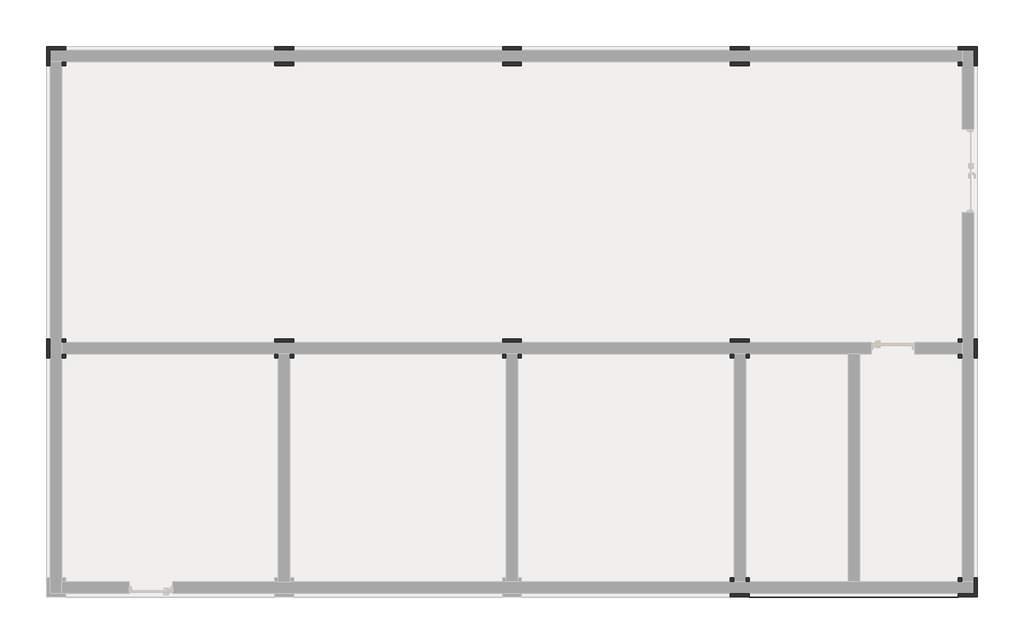
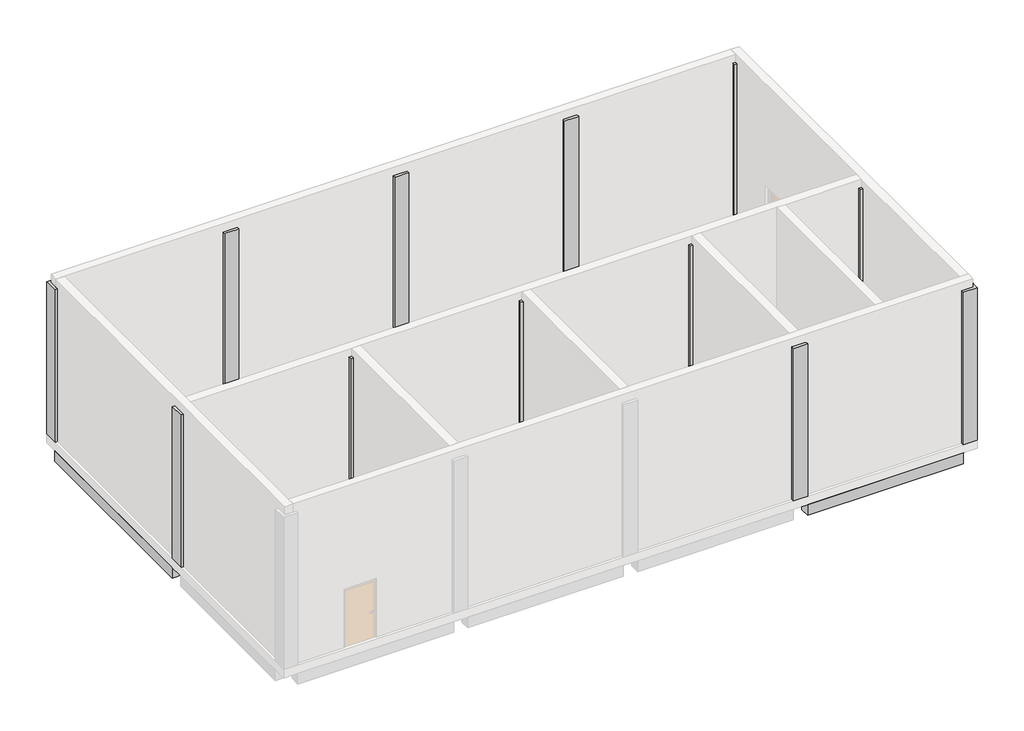
# One storey, part 2 of 2: 12 columns, 8 beams.
"""IFC4 building model written with IfcOpenShell, lengths in millimetres."""

import ifcopenshell
import ifcopenshell.guid

model = None  # the IFC model being written
_history = None  # IfcOwnerHistory: only IFC2X3 demands one
_inside = {}  # id of a spatial element -> (the spatial element, [elements in it])
_under = {}  # id of a project, library or spatial element -> (it, [spatial elements below it])
_declared = {}  # id of a project -> (the project, [libraries it declares])
_typed = {}  # id of a type object -> (the type object, [elements of that type])
_made_of = {}  # id of a material, layer set ... -> (it, [elements and type objects made of it])


def new_model(schema):
    """Start an empty IFC model of exactly this schema.

    Asked for "IFC4X3", IfcOpenShell would pick the latest addendum, in which some entities
    have other attributes; the version numbers below select the first issue.
    IFC2X3 requires an IfcOwnerHistory on every rooted entity: one is made here for all.
    """
    global model, _history
    if schema == "IFC4X3":
        model = ifcopenshell.file(schema_version=(4, 3, 0, 0))
    else:
        model = ifcopenshell.file(schema=schema)
    _inside.clear()
    _under.clear()
    _declared.clear()
    _typed.clear()
    _made_of.clear()
    _history = None
    if model.schema == "IFC2X3":
        org = make("IfcOrganization", Name="unknown")
        user = make(
            "IfcPersonAndOrganization",
            ThePerson=make("IfcPerson", FamilyName="unknown"),
            TheOrganization=org,
        )
        app = make(
            "IfcApplication",
            ApplicationDeveloper=org,
            Version="unknown",
            ApplicationFullName="unknown",
            ApplicationIdentifier="unknown",
        )
        _history = make(
            "IfcOwnerHistory",
            OwningUser=user,
            OwningApplication=app,
            ChangeAction="ADDED",
            CreationDate=0,
        )
    return model


def make(cls, **values):
    """One entity of the class cls with the attributes given. An attribute that is None is left unset."""
    return model.create_entity(
        cls, **{name: value for name, value in values.items() if value is not None}
    )


def rooted(cls, **values):
    """An entity with a GlobalId (a new one), such as an element, a storey or a relation."""
    return make(cls, GlobalId=ifcopenshell.guid.new(), OwnerHistory=_history, **values)


def si_unit(unit_type, name, prefix=None):
    """IfcSIUnit, for example si_unit("LENGTHUNIT", "METRE", prefix="MILLI")."""
    return make("IfcSIUnit", UnitType=unit_type, Prefix=prefix, Name=name)


def assignment(units):
    """IfcUnitAssignment: the units of a project."""
    return None if units is None else make("IfcUnitAssignment", Units=units)


def point(xyz):
    """IfcCartesianPoint."""
    return None if xyz is None else make("IfcCartesianPoint", Coordinates=xyz)


def direction(xyz):
    """IfcDirection."""
    return None if xyz is None else make("IfcDirection", DirectionRatios=xyz)


def frame(location, z_axis=None, x_axis=None):
    """IfcAxis2Placement3D, a coordinate frame: its origin and axes. An axis left out is left unset."""
    return make(
        "IfcAxis2Placement3D",
        Location=point(location),
        Axis=direction(z_axis),
        RefDirection=direction(x_axis),
    )


def origin():
    """The frame at (0, 0, 0) with its axes left unset."""
    return frame((0.0, 0.0, 0.0))


def place(relative_to, where):
    """IfcLocalPlacement: puts the frame where relative to a parent placement (None: the world)."""
    return make(
        "IfcLocalPlacement", PlacementRelTo=relative_to, RelativePlacement=where
    )


def context(
    kind, dimensions, precision=None, world=None, true_north=None, identifier=None
):
    """IfcGeometricRepresentationContext, for example the 3D "Model" context."""
    return make(
        "IfcGeometricRepresentationContext",
        ContextIdentifier=identifier,
        ContextType=kind,
        CoordinateSpaceDimension=dimensions,
        Precision=precision,
        WorldCoordinateSystem=world,
        TrueNorth=true_north,
    )


def project(units=None, contexts=None):
    """IfcProject with its units and contexts."""
    return rooted(
        "IfcProject",
        Name="project",
        RepresentationContexts=contexts,
        UnitsInContext=assignment(units),
    )


def spatial(cls, under=None, at=None, **own):
    """A site, building, storey or space (cls), placed at a placement, below another one or the project."""
    s = rooted(cls, ObjectPlacement=at, **own)
    if under is not None:
        _under.setdefault(under.id(), (under, []))[1].append(s)
    return s


def polyline(points):
    """IfcPolyline through the points."""
    return make("IfcPolyline", Points=[point(p) for p in points])


def outline(outer, holes=None, kind="AREA"):
    """IfcArbitraryClosedProfileDef: a profile drawn as a closed curve; with holes, ...WithVoids."""
    if holes is None:
        return make("IfcArbitraryClosedProfileDef", ProfileType=kind, OuterCurve=outer)
    return make(
        "IfcArbitraryProfileDefWithVoids",
        ProfileType=kind,
        OuterCurve=outer,
        InnerCurves=holes,
    )


def extrude(swept, where, along, depth):
    """IfcExtrudedAreaSolid: the profile swept, set in the frame where, extruded along a direction by depth."""
    return make(
        "IfcExtrudedAreaSolid",
        SweptArea=swept,
        Position=where,
        ExtrudedDirection=direction(along),
        Depth=depth,
    )


def faces_of(points, faces, orient=None, outer=None):
    """IfcFace entities. A face is a list of loops; a loop is a list of indices into points, from 0.

    orient and outer hold one flag for each loop. By default every Orientation is true, the
    first loop of a face is its IfcFaceOuterBound and the others are IfcFaceBound.
    """
    made = []
    for i, loops in enumerate(faces):
        bounds = []
        for j, loop in enumerate(loops):
            is_outer = j == 0 if outer is None else outer[i][j]
            bounds.append(
                make(
                    "IfcFaceOuterBound" if is_outer else "IfcFaceBound",
                    Bound=make("IfcPolyLoop", Polygon=[points[k] for k in loop]),
                    Orientation=True if orient is None else orient[i][j],
                )
            )
        made.append(make("IfcFace", Bounds=bounds))
    return made


def faceted_brep(points, faces, orient=None, outer=None, voids=None):
    """IfcFacetedBrep: a solid bounded by flat faces; with voids (closed shells), ...WithVoids."""
    shared = [point(p) for p in points]
    hull = make("IfcClosedShell", CfsFaces=faces_of(shared, faces, orient, outer))
    if voids is None:
        return make("IfcFacetedBrep", Outer=hull)
    return make(
        "IfcFacetedBrepWithVoids",
        Outer=hull,
        Voids=[
            make(cls, CfsFaces=faces_of(shared, fs, o, b)) for cls, fs, o, b in voids
        ],
    )


def shape(context_of_items, identifier, shape_type, items):
    """IfcShapeRepresentation: the items that make up one representation, for example the "Body"."""
    return make(
        "IfcShapeRepresentation",
        ContextOfItems=context_of_items,
        RepresentationIdentifier=identifier,
        RepresentationType=shape_type,
        Items=items,
    )


def made_of(thing, what):
    """Note that an element or type object is made of a material, layer set ...; save() writes the relation."""
    if what is not None:
        _made_of.setdefault(what.id(), (what, []))[1].append(thing)
    return thing


def element(
    cls,
    number,
    at=None,
    inside=None,
    cuts=None,
    type_object=None,
    material=None,
    context=None,
    identifier="Body",
    shape_type=None,
    held_by="IfcProductDefinitionShape",
    body=None,
    shapes=None,
    **own,
):
    """One element of the class cls, such as IfcWall. Its Tag is "e" and its number.

    at: its placement. inside: the storey or other place that contains it. cuts: it is an
    opening in that element (IfcRelVoidsElement). A single representation is given by context,
    identifier, shape_type and body (its items); several are given by shapes. held_by: the class
    of the entity that holds the representations. save() writes the other relations.
    """
    e = rooted(cls, Tag="e%d" % number, ObjectPlacement=at, **own)
    if body is not None:
        shapes = [shape(context, identifier, shape_type, body)]
    if shapes is not None:
        e.Representation = make(held_by, Representations=shapes)
    if inside is not None:
        _inside.setdefault(inside.id(), (inside, []))[1].append(e)
    if cuts is not None:
        rooted(
            "IfcRelVoidsElement", RelatingBuildingElement=cuts, RelatedOpeningElement=e
        )
    if type_object is not None:
        _typed.setdefault(type_object.id(), (type_object, []))[1].append(e)
    return made_of(e, material)


def aggregate(whole, parts):
    """IfcRelAggregates: a whole, such as a stair, and the parts it consists of."""
    return rooted("IfcRelAggregates", RelatingObject=whole, RelatedObjects=parts)


def save(model, path):
    """Write the relations noted so far, then the file.

    IfcRelAggregates (storeys below a building ...), IfcRelContainedInSpatialStructure (elements
    in a storey), IfcRelDefinesByType, IfcRelAssociatesMaterial and IfcRelDeclares: one each for
    every whole, place, type object, material and project.
    """
    for whole, parts in _under.values():
        aggregate(whole, parts)
    for where, things in _inside.values():
        rooted(
            "IfcRelContainedInSpatialStructure",
            RelatedElements=things,
            RelatingStructure=where,
        )
    for kind, things in _typed.values():
        rooted("IfcRelDefinesByType", RelatedObjects=things, RelatingType=kind)
    for what, things in _made_of.values():
        rooted("IfcRelAssociatesMaterial", RelatedObjects=things, RelatingMaterial=what)
    for by, libraries in _declared.values():
        rooted("IfcRelDeclares", RelatingContext=by, RelatedDefinitions=libraries)
    model.write(path)


model = new_model("IFC4")

# Units and contexts
model_context = context("Model", 3, world=origin())
ifc_project = project(units=[si_unit("LENGTHUNIT", "METRE", prefix="MILLI")], contexts=[model_context])

# Site, building, storey
site = spatial("IfcSite", under=ifc_project)
building = spatial("IfcBuilding", under=site)
storey = spatial("IfcBuildingStorey", under=building, Name="1st FL GL+200", Elevation=0.0)

# Beams
placement = place(None, origin())
element("IfcBeam", 1, ObjectType="RC Beam_Rectangular : 350 x 700mm", at=placement, inside=storey, context=model_context, shape_type="SweptSolid", body=[
    extrude(outline(polyline([(5204.2726763, 1485.9763125), (5554.2726763, 1485.9763125), (5554.2726763, -4314.0236875), (5204.2726763, -4314.0236875), (5204.2726763, 1485.9763125)])), frame((0.0, 0.0, -700.0), z_axis=(0.0, 0.0, 1.0), x_axis=(1.0, 0.0, 0.0)), (0.0, 0.0, 1.0), 400.0),
])
element("IfcBeam", 2, ObjectType="RC Beam_Rectangular : 350 x 700mm", at=placement, inside=storey, context=model_context, shape_type="SweptSolid", body=[
    extrude(outline(polyline([(5554.2726763, 1998.6763125), (5204.2726763, 1998.6763125), (5204.2726763, 9185.9763125), (5554.2726763, 9185.9763125), (5554.2726763, 1998.6763125)])), frame((0.0, 0.0, -700.0), z_axis=(0.0, 0.0, 1.0), x_axis=(1.0, 0.0, 0.0)), (0.0, 0.0, 1.0), 400.0),
])
element("IfcBeam", 3, ObjectType="RC Beam_Rectangular : 350 x 700mm", at=placement, inside=storey, context=model_context, shape_type="SweptSolid", body=[
    extrude(outline(polyline([(-18595.7273237, 1998.6763125), (-18945.7273237, 1998.6763125), (-18945.7273237, 9185.9763125), (-18595.7273237, 9185.9763125), (-18595.7273237, 1998.6763125)])), frame((0.0, 0.0, -700.0), z_axis=(0.0, 0.0, 1.0), x_axis=(1.0, 0.0, 0.0)), (0.0, 0.0, 1.0), 400.0),
])
element("IfcBeam", 4, ObjectType="RC Beam_Rectangular : 350 x 700mm", at=placement, inside=storey, context=model_context, shape_type="SweptSolid", body=[
    extrude(outline(polyline([(-12945.7273237, 9685.9763125), (-12945.7273237, 9335.9763125), (-18445.7273237, 9335.9763125), (-18445.7273237, 9685.9763125), (-12945.7273237, 9685.9763125)])), frame((0.0, 0.0, -700.0), z_axis=(0.0, 0.0, 1.0), x_axis=(1.0, 0.0, 0.0)), (0.0, 0.0, 1.0), 400.0),
])
element("IfcBeam", 5, ObjectType="RC Beam_Rectangular : 350 x 700mm", at=placement, inside=storey, context=model_context, shape_type="SweptSolid", body=[
    extrude(outline(polyline([(-12433.0273237, 9335.9763125), (-12433.0273237, 9685.9763125), (-6945.7273237, 9685.9763125), (-6945.7273237, 9335.9763125), (-12433.0273237, 9335.9763125)])), frame((0.0, 0.0, -700.0), z_axis=(0.0, 0.0, 1.0), x_axis=(1.0, 0.0, 0.0)), (0.0, 0.0, 1.0), 400.0),
])
element("IfcBeam", 6, ObjectType="RC Beam_Rectangular : 350 x 700mm", at=placement, inside=storey, context=model_context, shape_type="SweptSolid", body=[
    extrude(outline(polyline([(-6433.0273237, 9335.9763125), (-6433.0273237, 9685.9763125), (-945.7273237, 9685.9763125), (-945.7273237, 9335.9763125), (-6433.0273237, 9335.9763125)])), frame((0.0, 0.0, -700.0), z_axis=(0.0, 0.0, 1.0), x_axis=(1.0, 0.0, 0.0)), (0.0, 0.0, 1.0), 400.0),
])
element("IfcBeam", 7, ObjectType="RC Beam_Rectangular : 350 x 700mm", at=placement, inside=storey, context=model_context, shape_type="SweptSolid", body=[
    extrude(outline(polyline([(-433.0273237, 9335.9763125), (-433.0273237, 9685.9763125), (5054.2726763, 9685.9763125), (5054.2726763, 9335.9763125), (-433.0273237, 9335.9763125)])), frame((0.0, 0.0, -700.0), z_axis=(0.0, 0.0, 1.0), x_axis=(1.0, 0.0, 0.0)), (0.0, 0.0, 1.0), 400.0),
])
element("IfcBeam", 8, ObjectType="RC Beam_Rectangular : 350 x 700mm", at=placement, inside=storey, context=model_context, shape_type="SweptSolid", body=[
    extrude(outline(polyline([(5054.2726763, -4464.0236875), (5054.2726763, -4814.0236875), (-445.7273237, -4814.0236875), (-445.7273237, -4464.0236875), (5054.2726763, -4464.0236875)])), frame((0.0, 0.0, -700.0), z_axis=(0.0, 0.0, 1.0), x_axis=(1.0, 0.0, 0.0)), (0.0, 0.0, 1.0), 400.0),
])

# Columns
element("IfcColumn", 9, ObjectType="RC_Column_Rectangular : 500 x 500mm", at=placement, inside=storey, context=model_context, shape_type="Brep", body=[
    faceted_brep([(-18945.7273237, 9185.9763125, 0.0), (-18945.7273237, 9685.9763125, 0.0), (-18445.7273237, 9685.9763125, 0.0), (-18445.7273237, 9585.9763125, 0.0), (-18845.7273237, 9585.9763125, 0.0), (-18845.7273237, 9285.9763125, 0.0), (-18845.7273237, 9185.9763125, 0.0), (-18945.7273237, 9685.9763125, 5700.0), (-18445.7273237, 9685.9763125, 5700.0), (-18445.7273237, 9685.9763125, 5300.0), (-18945.7273237, 9185.9763125, 5300.0), (-18945.7273237, 9185.9763125, 5700.0), (-18845.7273237, 9185.9763125, 5300.0), (-18845.7273237, 9185.9763125, 5700.0), (-18445.7273237, 9585.9763125, 5700.0), (-18445.7273237, 9585.9763125, 5300.0), (-18845.7273237, 9585.9763125, 5700.0)], [[[0, 1, 2, 3, 4, 5, 6]], [[2, 1, 7, 8, 9]], [[1, 0, 10, 11, 7]], [[11, 10, 0, 6, 12, 13]], [[2, 9, 8, 14, 15, 3]], [[16, 4, 3, 15, 14]], [[4, 16, 13, 12, 6, 5]], [[8, 7, 11, 13, 16, 14]]]),
    faceted_brep([(-18445.7273237, 9185.9763125, 5700.0), (-18445.7273237, 9285.9763125, 5700.0), (-18545.7273237, 9285.9763125, 5700.0), (-18545.7273237, 9185.9763125, 5700.0), (-18445.7273237, 9285.9763125, 0.0), (-18545.7273237, 9285.9763125, 0.0), (-18445.7273237, 9185.9763125, 0.0), (-18545.7273237, 9185.9763125, 0.0)], [[[0, 1, 2, 3]], [[1, 4, 5, 2]], [[0, 6, 4, 1]], [[5, 7, 3, 2]], [[4, 6, 7, 5]], [[6, 0, 3, 7]]]),
])
element("IfcColumn", 10, ObjectType="RC_Column_Rectangular : 500 x 500mm", at=placement, inside=storey, context=model_context, shape_type="Brep", body=[
    faceted_brep([(-18945.7273237, 1485.9763125, 0.0), (-18945.7273237, 1985.9763125, 0.0), (-18845.7273237, 1985.9763125, 0.0), (-18845.7273237, 1485.9763125, 0.0), (-18945.7273237, 1485.9763125, 5300.0), (-18945.7273237, 1485.9763125, 5700.0), (-18945.7273237, 1985.9763125, 5700.0), (-18945.7273237, 1985.9763125, 5300.0), (-18845.7273237, 1485.9763125, 5300.0), (-18845.7273237, 1485.9763125, 5700.0), (-18845.7273237, 1985.9763125, 5300.0), (-18845.7273237, 1985.9763125, 5700.0)], [[[0, 1, 2, 3]], [[1, 0, 4, 5, 6, 7]], [[5, 4, 0, 3, 8, 9]], [[3, 2, 10, 11, 9, 8]], [[1, 7, 6, 11, 10, 2]], [[6, 5, 9, 11]]]),
    faceted_brep([(-18445.7273237, 1985.9763125, 5700.0), (-18445.7273237, 1985.9763125, 0.0), (-18545.7273237, 1985.9763125, 0.0), (-18545.7273237, 1985.9763125, 5700.0), (-18445.7273237, 1910.9763125, 5700.0), (-18445.7273237, 1885.9763125, 5700.0), (-18445.7273237, 1885.9763125, 5300.0), (-18445.7273237, 1885.9763125, 0.0), (-18545.7273237, 1885.9763125, 0.0), (-18545.7273237, 1885.9763125, 5700.0)], [[[0, 1, 2, 3]], [[1, 0, 4, 5, 6, 7]], [[2, 1, 7, 8]], [[7, 6, 5, 9, 8]], [[0, 3, 9, 5, 4]], [[3, 2, 8, 9]]]),
    faceted_brep([(-18545.7273237, 1485.9763125, 5700.0), (-18445.7273237, 1485.9763125, 5700.0), (-18445.7273237, 1560.9763125, 5700.0), (-18445.7273237, 1585.9763125, 5700.0), (-18545.7273237, 1585.9763125, 5700.0), (-18545.7273237, 1485.9763125, 0.0), (-18545.7273237, 1585.9763125, 0.0), (-18445.7273237, 1485.9763125, 0.0), (-18445.7273237, 1585.9763125, 5300.0), (-18445.7273237, 1585.9763125, 0.0)], [[[0, 1, 2, 3, 4]], [[5, 0, 4, 6]], [[7, 1, 0, 5]], [[3, 8, 9, 6, 4]], [[1, 7, 9, 8, 3, 2]], [[7, 5, 6, 9]]]),
])
element("IfcColumn", 11, ObjectType="RC_Column_Rectangular : 500 x 500mm", at=placement, inside=storey, context=model_context, shape_type="Brep", body=[
    faceted_brep([(-12945.7273237, 9685.9763125, 0.0), (-12445.7273237, 9685.9763125, 0.0), (-12445.7273237, 9585.9763125, 0.0), (-12945.7273237, 9585.9763125, 0.0), (-12945.7273237, 9685.9763125, 5300.0), (-12945.7273237, 9685.9763125, 5700.0), (-12445.7273237, 9685.9763125, 5700.0), (-12945.7273237, 9585.9763125, 5300.0), (-12945.7273237, 9585.9763125, 5700.0), (-12445.7273237, 9585.9763125, 5700.0)], [[[0, 1, 2, 3]], [[1, 0, 4, 5, 6]], [[5, 4, 0, 3, 7, 8]], [[1, 6, 9, 2]], [[3, 2, 9, 8, 7]], [[6, 5, 8, 9]]]),
    faceted_brep([(-12945.7273237, 9185.9763125, 0.0), (-12445.7273237, 9185.9763125, 0.0), (-12445.7273237, 9185.9763125, 5700.0), (-12520.7273237, 9185.9763125, 5700.0), (-12870.7273237, 9185.9763125, 5700.0), (-12945.7273237, 9185.9763125, 5700.0), (-12445.7273237, 9285.9763125, 5700.0), (-12945.7273237, 9285.9763125, 5700.0), (-12445.7273237, 9285.9763125, 0.0), (-12945.7273237, 9285.9763125, 0.0)], [[[0, 1, 2, 3, 4, 5]], [[5, 4, 3, 2, 6, 7]], [[8, 9, 7, 6]], [[1, 0, 9, 8]], [[0, 5, 7, 9]], [[2, 1, 8, 6]]]),
])
element("IfcColumn", 12, ObjectType="RC_Column_Rectangular : 500 x 500mm", at=placement, inside=storey, context=model_context, shape_type="Brep", body=[
    faceted_brep([(-12945.7273237, 1985.9763125, 0.0), (-12445.7273237, 1985.9763125, 0.0), (-12445.7273237, 1885.9763125, 0.0), (-12945.7273237, 1885.9763125, 0.0), (-12945.7273237, 1985.9763125, 5700.0), (-12870.7273237, 1985.9763125, 5700.0), (-12520.7273237, 1985.9763125, 5700.0), (-12445.7273237, 1985.9763125, 5700.0), (-12945.7273237, 1885.9763125, 5300.0), (-12945.7273237, 1885.9763125, 5700.0), (-12945.7273237, 1910.9763125, 5700.0), (-12445.7273237, 1910.9763125, 5700.0), (-12445.7273237, 1885.9763125, 5700.0), (-12445.7273237, 1885.9763125, 5300.0)], [[[0, 1, 2, 3]], [[1, 0, 4, 5, 6, 7]], [[4, 0, 3, 8, 9, 10]], [[1, 7, 11, 12, 13, 2]], [[3, 2, 13, 12, 9, 8]], [[7, 6, 5, 4, 10, 9, 12, 11]]]),
    faceted_brep([(-12945.7273237, 1485.9763125, 5700.0), (-12945.7273237, 1485.9763125, 0.0), (-12845.7273237, 1485.9763125, 0.0), (-12845.7273237, 1485.9763125, 5300.0), (-12845.7273237, 1485.9763125, 5700.0), (-12870.7273237, 1485.9763125, 5700.0), (-12945.7273237, 1585.9763125, 0.0), (-12945.7273237, 1585.9763125, 5300.0), (-12945.7273237, 1585.9763125, 5700.0), (-12845.7273237, 1585.9763125, 5700.0), (-12845.7273237, 1585.9763125, 0.0), (-12945.7273237, 1560.9763125, 5700.0)], [[[0, 1, 2, 3, 4, 5]], [[6, 7, 8, 9, 10]], [[1, 6, 10, 2]], [[1, 0, 11, 8, 7, 6]], [[4, 3, 2, 10, 9]], [[8, 11, 0, 5, 4, 9]]]),
    faceted_brep([(-12445.7273237, 1485.9763125, 5700.0), (-12445.7273237, 1560.9763125, 5700.0), (-12445.7273237, 1585.9763125, 5700.0), (-12545.7273237, 1585.9763125, 5700.0), (-12545.7273237, 1485.9763125, 5700.0), (-12520.7273237, 1485.9763125, 5700.0), (-12445.7273237, 1485.9763125, 0.0), (-12445.7273237, 1585.9763125, 0.0), (-12445.7273237, 1585.9763125, 5300.0), (-12545.7273237, 1485.9763125, 0.0), (-12545.7273237, 1485.9763125, 5300.0), (-12545.7273237, 1585.9763125, 0.0)], [[[0, 1, 2, 3, 4, 5]], [[0, 6, 7, 8, 2, 1]], [[9, 10, 4, 3, 11]], [[6, 0, 5, 4, 10, 9]], [[2, 8, 7, 11, 3]], [[7, 6, 9, 11]]]),
])
element("IfcColumn", 13, ObjectType="RC_Column_Rectangular : 500 x 500mm", at=placement, inside=storey, context=model_context, shape_type="Brep", body=[
    faceted_brep([(-6945.7273237, 9685.9763125, 0.0), (-6445.7273237, 9685.9763125, 0.0), (-6445.7273237, 9585.9763125, 0.0), (-6945.7273237, 9585.9763125, 0.0), (-6945.7273237, 9685.9763125, 5300.0), (-6945.7273237, 9685.9763125, 5700.0), (-6445.7273237, 9685.9763125, 5700.0), (-6945.7273237, 9585.9763125, 5300.0), (-6945.7273237, 9585.9763125, 5700.0), (-6445.7273237, 9585.9763125, 5700.0)], [[[0, 1, 2, 3]], [[1, 0, 4, 5, 6]], [[5, 4, 0, 3, 7, 8]], [[1, 6, 9, 2]], [[3, 2, 9, 8, 7]], [[6, 5, 8, 9]]]),
    faceted_brep([(-6945.7273237, 9185.9763125, 0.0), (-6445.7273237, 9185.9763125, 0.0), (-6445.7273237, 9185.9763125, 5700.0), (-6520.7273237, 9185.9763125, 5700.0), (-6870.7273237, 9185.9763125, 5700.0), (-6945.7273237, 9185.9763125, 5700.0), (-6445.7273237, 9285.9763125, 5700.0), (-6945.7273237, 9285.9763125, 5700.0), (-6445.7273237, 9285.9763125, 0.0), (-6945.7273237, 9285.9763125, 0.0)], [[[0, 1, 2, 3, 4, 5]], [[5, 4, 3, 2, 6, 7]], [[8, 9, 7, 6]], [[1, 0, 9, 8]], [[0, 5, 7, 9]], [[2, 1, 8, 6]]]),
])
element("IfcColumn", 14, ObjectType="RC_Column_Rectangular : 500 x 500mm", at=placement, inside=storey, context=model_context, shape_type="Brep", body=[
    faceted_brep([(-6945.7273237, 1985.9763125, 0.0), (-6445.7273237, 1985.9763125, 0.0), (-6445.7273237, 1885.9763125, 0.0), (-6945.7273237, 1885.9763125, 0.0), (-6945.7273237, 1985.9763125, 5700.0), (-6870.7273237, 1985.9763125, 5700.0), (-6520.7273237, 1985.9763125, 5700.0), (-6445.7273237, 1985.9763125, 5700.0), (-6945.7273237, 1885.9763125, 5300.0), (-6945.7273237, 1885.9763125, 5700.0), (-6945.7273237, 1910.9763125, 5700.0), (-6445.7273237, 1910.9763125, 5700.0), (-6445.7273237, 1885.9763125, 5700.0), (-6445.7273237, 1885.9763125, 5300.0)], [[[0, 1, 2, 3]], [[1, 0, 4, 5, 6, 7]], [[4, 0, 3, 8, 9, 10]], [[1, 7, 11, 12, 13, 2]], [[3, 2, 13, 12, 9, 8]], [[7, 6, 5, 4, 10, 9, 12, 11]]]),
    faceted_brep([(-6945.7273237, 1485.9763125, 5700.0), (-6945.7273237, 1485.9763125, 0.0), (-6845.7273237, 1485.9763125, 0.0), (-6845.7273237, 1485.9763125, 5300.0), (-6845.7273237, 1485.9763125, 5700.0), (-6870.7273237, 1485.9763125, 5700.0), (-6945.7273237, 1585.9763125, 0.0), (-6945.7273237, 1585.9763125, 5300.0), (-6945.7273237, 1585.9763125, 5700.0), (-6845.7273237, 1585.9763125, 5700.0), (-6845.7273237, 1585.9763125, 0.0), (-6945.7273237, 1560.9763125, 5700.0)], [[[0, 1, 2, 3, 4, 5]], [[6, 7, 8, 9, 10]], [[1, 6, 10, 2]], [[1, 0, 11, 8, 7, 6]], [[4, 3, 2, 10, 9]], [[8, 11, 0, 5, 4, 9]]]),
    faceted_brep([(-6445.7273237, 1485.9763125, 5700.0), (-6445.7273237, 1560.9763125, 5700.0), (-6445.7273237, 1585.9763125, 5700.0), (-6545.7273237, 1585.9763125, 5700.0), (-6545.7273237, 1485.9763125, 5700.0), (-6520.7273237, 1485.9763125, 5700.0), (-6445.7273237, 1485.9763125, 0.0), (-6445.7273237, 1585.9763125, 0.0), (-6445.7273237, 1585.9763125, 5300.0), (-6545.7273237, 1485.9763125, 0.0), (-6545.7273237, 1485.9763125, 5300.0), (-6545.7273237, 1585.9763125, 0.0)], [[[0, 1, 2, 3, 4, 5]], [[0, 6, 7, 8, 2, 1]], [[9, 10, 4, 3, 11]], [[6, 0, 5, 4, 10, 9]], [[2, 8, 7, 11, 3]], [[7, 6, 9, 11]]]),
])
element("IfcColumn", 15, ObjectType="RC_Column_Rectangular : 500 x 500mm", at=placement, inside=storey, context=model_context, shape_type="Brep", body=[
    faceted_brep([(-945.7273237, 9685.9763125, 0.0), (-445.7273237, 9685.9763125, 0.0), (-445.7273237, 9585.9763125, 0.0), (-945.7273237, 9585.9763125, 0.0), (-945.7273237, 9685.9763125, 5300.0), (-945.7273237, 9685.9763125, 5700.0), (-445.7273237, 9685.9763125, 5700.0), (-945.7273237, 9585.9763125, 5300.0), (-945.7273237, 9585.9763125, 5700.0), (-445.7273237, 9585.9763125, 5700.0)], [[[0, 1, 2, 3]], [[1, 0, 4, 5, 6]], [[5, 4, 0, 3, 7, 8]], [[1, 6, 9, 2]], [[3, 2, 9, 8, 7]], [[6, 5, 8, 9]]]),
    faceted_brep([(-945.7273237, 9185.9763125, 0.0), (-445.7273237, 9185.9763125, 0.0), (-445.7273237, 9185.9763125, 5700.0), (-520.7273237, 9185.9763125, 5700.0), (-870.7273237, 9185.9763125, 5700.0), (-945.7273237, 9185.9763125, 5700.0), (-445.7273237, 9285.9763125, 5700.0), (-945.7273237, 9285.9763125, 5700.0), (-445.7273237, 9285.9763125, 0.0), (-945.7273237, 9285.9763125, 0.0)], [[[0, 1, 2, 3, 4, 5]], [[5, 4, 3, 2, 6, 7]], [[8, 9, 7, 6]], [[1, 0, 9, 8]], [[0, 5, 7, 9]], [[2, 1, 8, 6]]]),
])
element("IfcColumn", 16, ObjectType="RC_Column_Rectangular : 500 x 500mm", at=placement, inside=storey, context=model_context, shape_type="Brep", body=[
    faceted_brep([(-945.7273237, 1985.9763125, 0.0), (-445.7273237, 1985.9763125, 0.0), (-445.7273237, 1885.9763125, 0.0), (-945.7273237, 1885.9763125, 0.0), (-945.7273237, 1985.9763125, 5700.0), (-870.7273237, 1985.9763125, 5700.0), (-520.7273237, 1985.9763125, 5700.0), (-445.7273237, 1985.9763125, 5700.0), (-945.7273237, 1885.9763125, 5300.0), (-945.7273237, 1885.9763125, 5700.0), (-945.7273237, 1910.9763125, 5700.0), (-445.7273237, 1910.9763125, 5700.0), (-445.7273237, 1885.9763125, 5700.0), (-445.7273237, 1885.9763125, 5300.0)], [[[0, 1, 2, 3]], [[1, 0, 4, 5, 6, 7]], [[4, 0, 3, 8, 9, 10]], [[1, 7, 11, 12, 13, 2]], [[3, 2, 13, 12, 9, 8]], [[7, 6, 5, 4, 10, 9, 12, 11]]]),
    faceted_brep([(-945.7273237, 1485.9763125, 5700.0), (-945.7273237, 1485.9763125, 0.0), (-845.7273237, 1485.9763125, 0.0), (-845.7273237, 1485.9763125, 5300.0), (-845.7273237, 1485.9763125, 5700.0), (-870.7273237, 1485.9763125, 5700.0), (-945.7273237, 1585.9763125, 0.0), (-945.7273237, 1585.9763125, 5300.0), (-945.7273237, 1585.9763125, 5700.0), (-845.7273237, 1585.9763125, 5700.0), (-845.7273237, 1585.9763125, 0.0), (-945.7273237, 1560.9763125, 5700.0)], [[[0, 1, 2, 3, 4, 5]], [[6, 7, 8, 9, 10]], [[1, 6, 10, 2]], [[1, 0, 11, 8, 7, 6]], [[4, 3, 2, 10, 9]], [[8, 11, 0, 5, 4, 9]]]),
    faceted_brep([(-445.7273237, 1485.9763125, 5700.0), (-445.7273237, 1560.9763125, 5700.0), (-445.7273237, 1585.9763125, 5700.0), (-545.7273237, 1585.9763125, 5700.0), (-545.7273237, 1485.9763125, 5700.0), (-520.7273237, 1485.9763125, 5700.0), (-445.7273237, 1485.9763125, 0.0), (-445.7273237, 1585.9763125, 0.0), (-445.7273237, 1585.9763125, 5300.0), (-545.7273237, 1485.9763125, 0.0), (-545.7273237, 1485.9763125, 5300.0), (-545.7273237, 1585.9763125, 0.0)], [[[0, 1, 2, 3, 4, 5]], [[0, 6, 7, 8, 2, 1]], [[9, 10, 4, 3, 11]], [[6, 0, 5, 4, 10, 9]], [[2, 8, 7, 11, 3]], [[7, 6, 9, 11]]]),
])
element("IfcColumn", 17, ObjectType="RC_Column_Rectangular : 500 x 500mm", at=placement, inside=storey, context=model_context, shape_type="Brep", body=[
    faceted_brep([(-945.7273237, -4414.0236875, 0.0), (-945.7273237, -4314.0236875, 0.0), (-845.7273237, -4314.0236875, 0.0), (-845.7273237, -4414.0236875, 0.0), (-945.7273237, -4314.0236875, 5700.0), (-945.7273237, -4414.0236875, 5700.0), (-845.7273237, -4314.0236875, 5300.0), (-845.7273237, -4314.0236875, 5700.0), (-845.7273237, -4414.0236875, 5700.0), (-870.7273237, -4314.0236875, 5700.0)], [[[0, 1, 2, 3]], [[4, 1, 0, 5]], [[3, 2, 6, 7, 8]], [[1, 4, 9, 7, 6, 2]], [[5, 0, 3, 8]], [[4, 5, 8, 7, 9]]]),
    faceted_brep([(-445.7273237, -4314.0236875, 5700.0), (-445.7273237, -4314.0236875, 0.0), (-545.7273237, -4314.0236875, 0.0), (-545.7273237, -4314.0236875, 5300.0), (-545.7273237, -4314.0236875, 5700.0), (-520.7273237, -4314.0236875, 5700.0), (-445.7273237, -4414.0236875, 5700.0), (-445.7273237, -4414.0236875, 0.0), (-545.7273237, -4414.0236875, 5700.0), (-545.7273237, -4414.0236875, 0.0)], [[[0, 1, 2, 3, 4, 5]], [[1, 0, 6, 7]], [[7, 6, 8, 9]], [[6, 0, 5, 4, 8]], [[2, 9, 8, 4, 3]], [[1, 7, 9, 2]]]),
    faceted_brep([(-945.7273237, -4814.0236875, 0.0), (-445.7273237, -4814.0236875, 0.0), (-445.7273237, -4814.0236875, 5300.0), (-445.7273237, -4814.0236875, 5700.0), (-945.7273237, -4814.0236875, 5700.0), (-945.7273237, -4814.0236875, 5300.0), (-445.7273237, -4714.0236875, 5700.0), (-945.7273237, -4714.0236875, 5700.0), (-445.7273237, -4714.0236875, 0.0), (-945.7273237, -4714.0236875, 0.0), (-945.7273237, -4714.0236875, 5300.0), (-445.7273237, -4714.0236875, 5300.0)], [[[0, 1, 2, 3, 4, 5]], [[4, 3, 6, 7]], [[8, 9, 10, 7, 6, 11]], [[1, 0, 9, 8]], [[0, 5, 4, 7, 10, 9]], [[3, 2, 1, 8, 11, 6]]]),
])
element("IfcColumn", 18, ObjectType="RC_Column_Rectangular : 500 x 500mm", at=placement, inside=storey, context=model_context, shape_type="Brep", body=[
    faceted_brep([(5054.2726763, 9185.9763125, 0.0), (5054.2726763, 9285.9763125, 0.0), (5154.2726763, 9285.9763125, 0.0), (5154.2726763, 9185.9763125, 0.0), (5054.2726763, 9185.9763125, 5700.0), (5154.2726763, 9185.9763125, 5700.0), (5054.2726763, 9285.9763125, 5700.0), (5154.2726763, 9285.9763125, 5700.0)], [[[0, 1, 2, 3]], [[4, 0, 3, 5]], [[6, 4, 5, 7]], [[2, 1, 6, 7]], [[0, 4, 6, 1]], [[3, 2, 7, 5]]]),
    faceted_brep([(5554.2726763, 9685.9763125, 0.0), (5054.2726763, 9685.9763125, 0.0), (5054.2726763, 9685.9763125, 5300.0), (5054.2726763, 9685.9763125, 5700.0), (5554.2726763, 9685.9763125, 5700.0), (5054.2726763, 9585.9763125, 0.0), (5054.2726763, 9585.9763125, 5300.0), (5054.2726763, 9585.9763125, 5700.0), (5554.2726763, 9185.9763125, 0.0), (5554.2726763, 9185.9763125, 5700.0), (5554.2726763, 9185.9763125, 5300.0), (5454.2726763, 9585.9763125, 0.0), (5454.2726763, 9585.9763125, 5700.0), (5154.2726763, 9585.9763125, 0.0), (5454.2726763, 9185.9763125, 0.0), (5454.2726763, 9185.9763125, 5300.0), (5454.2726763, 9185.9763125, 5700.0)], [[[0, 1, 2, 3, 4]], [[3, 2, 1, 5, 6, 7]], [[8, 0, 4, 9, 10]], [[11, 12, 7, 6, 5, 13]], [[12, 11, 14, 15, 16]], [[0, 8, 14, 11, 13, 5, 1]], [[8, 10, 9, 16, 15, 14]], [[4, 3, 7, 12, 16, 9]]]),
])
element("IfcColumn", 19, ObjectType="RC_Column_Rectangular : 500 x 500mm", at=placement, inside=storey, context=model_context, shape_type="Brep", body=[
    faceted_brep([(5054.2726763, 1985.9763125, 0.0), (5154.2726763, 1985.9763125, 0.0), (5154.2726763, 1885.9763125, 0.0), (5054.2726763, 1885.9763125, 0.0), (5054.2726763, 1985.9763125, 5700.0), (5054.2726763, 1885.9763125, 5300.0), (5054.2726763, 1885.9763125, 5700.0), (5054.2726763, 1910.9763125, 5700.0), (5154.2726763, 1985.9763125, 5700.0), (5154.2726763, 1885.9763125, 5700.0)], [[[0, 1, 2, 3]], [[4, 0, 3, 5, 6, 7]], [[1, 8, 9, 2]], [[0, 4, 8, 1]], [[3, 2, 9, 6, 5]], [[8, 4, 7, 6, 9]]]),
    faceted_brep([(5554.2726763, 1985.9763125, 5700.0), (5554.2726763, 1985.9763125, 0.0), (5454.2726763, 1985.9763125, 0.0), (5454.2726763, 1985.9763125, 5700.0), (5554.2726763, 1485.9763125, 0.0), (5554.2726763, 1485.9763125, 5700.0), (5554.2726763, 1485.9763125, 5300.0), (5454.2726763, 1485.9763125, 5700.0), (5454.2726763, 1485.9763125, 0.0), (5454.2726763, 1485.9763125, 5300.0)], [[[0, 1, 2, 3]], [[4, 1, 0, 5, 6]], [[5, 0, 3, 7]], [[2, 8, 9, 7, 3]], [[1, 4, 8, 2]], [[4, 6, 5, 7, 9, 8]]]),
    faceted_brep([(5054.2726763, 1485.9763125, 5700.0), (5054.2726763, 1485.9763125, 0.0), (5154.2726763, 1485.9763125, 0.0), (5154.2726763, 1485.9763125, 5700.0), (5154.2726763, 1585.9763125, 5700.0), (5054.2726763, 1585.9763125, 5700.0), (5054.2726763, 1560.9763125, 5700.0), (5154.2726763, 1585.9763125, 0.0), (5054.2726763, 1585.9763125, 0.0), (5054.2726763, 1585.9763125, 5300.0)], [[[0, 1, 2, 3]], [[0, 3, 4, 5, 6]], [[7, 8, 9, 5, 4]], [[2, 1, 8, 7]], [[1, 0, 6, 5, 9, 8]], [[3, 2, 7, 4]]]),
])
element("IfcColumn", 20, ObjectType="RC_Column_Rectangular : 500 x 500mm", at=placement, inside=storey, context=model_context, shape_type="Brep", body=[
    faceted_brep([(5054.2726763, -4414.0236875, 0.0), (5054.2726763, -4314.0236875, 0.0), (5154.2726763, -4314.0236875, 0.0), (5154.2726763, -4414.0236875, 0.0), (5054.2726763, -4314.0236875, 5700.0), (5054.2726763, -4414.0236875, 5700.0), (5154.2726763, -4414.0236875, 5700.0), (5154.2726763, -4314.0236875, 5700.0)], [[[0, 1, 2, 3]], [[4, 1, 0, 5]], [[5, 0, 3, 6]], [[3, 2, 7, 6]], [[1, 4, 7, 2]], [[4, 5, 6, 7]]]),
    faceted_brep([(5554.2726763, -4314.0236875, 5700.0), (5554.2726763, -4314.0236875, 5300.0), (5554.2726763, -4314.0236875, 0.0), (5454.2726763, -4314.0236875, 0.0), (5454.2726763, -4314.0236875, 5300.0), (5454.2726763, -4314.0236875, 5700.0), (5054.2726763, -4814.0236875, 0.0), (5554.2726763, -4814.0236875, 0.0), (5554.2726763, -4814.0236875, 5700.0), (5054.2726763, -4814.0236875, 5700.0), (5054.2726763, -4814.0236875, 5300.0), (5454.2726763, -4714.0236875, 5700.0), (5054.2726763, -4714.0236875, 5700.0), (5454.2726763, -4714.0236875, 0.0), (5054.2726763, -4714.0236875, 0.0), (5054.2726763, -4714.0236875, 5300.0), (5454.2726763, -4414.0236875, 0.0)], [[[0, 1, 2, 3, 4, 5]], [[6, 7, 8, 9, 10]], [[7, 2, 1, 0, 8]], [[9, 8, 0, 5, 11, 12]], [[11, 13, 14, 15, 12]], [[13, 11, 5, 4, 3, 16]], [[6, 10, 9, 12, 15, 14]], [[2, 7, 6, 14, 13, 16, 3]]]),
])

save(model, "model.ifc")

# Revit data of these elements
# Project information
#   Project Issue Date = "발행 날짜"
#   Project Status = "프로젝트 상태"
#   Client Name = "소유자"
#   Project Address = "주소를 여기에 입력"
#   Project Name = "프로젝트 이름"
#   Project Number = "0001"
#   AreaCalculationInternationalBuildNumber = "ZgA=BAAAAA==2023BgFlAAAAAQgAAAABAQAAAAYBZAAAAAHnBwAABAQAAAABUAQAAAcH0"
#   BuildingbookInternationalBuildNumber = "ZgA=BAAAAA==2023BgFlAAAAAQoAAAABAQAAAAYBZAAAAAHnBwAABAQAAAABWwIAAAcH0"
#   RoomBookInternationalBuildNumber = "ZgA=BAAAAA==2023BgFlAAAAAQQAAAABAQAAAAYBZAAAAAHnBwAABAQAAAABTwQAAAcH1"
# Grids (mm)
#   "X2": line (-12695.727, -8233.19) -> (-12695.727, 14438.726)
#   "X3": line (-6695.727, -8233.19) -> (-6695.727, 14438.726)
#   "X4": line (-695.727, -8233.19) -> (-695.727, 14438.726)
#   "X5": line (5304.273, -8233.19) -> (5304.273, 14438.726)
#   "Y2": line (9794.388, 1735.976) -> (-24604.07, 1735.976)
#   "Y1": line (9794.388, -4564.024) -> (-24604.07, -4564.024)
#   "Y3": line (9794.388, 9435.976) -> (-24604.07, 9435.976)
#   "X1": line (-18695.727, -8233.19) -> (-18695.727, 14438.726)
#   "Y61": line (2304.273, -8233.19) -> (2304.273, 3037.902)
#   "Y62": line (9794.388, 4135.976) -> (-10544.455, 4135.976)
#   "Y63": line (-9695.727, 3037.902) -> (-9695.727, 14438.726)
# Type "RC Beam_Rectangular : 350 x 700mm"
#   Length [instance default] = 1524 mm
#   b = 350 mm
#   h = 700 mm
#   Structural Material [instance default] = 콘크리트, 현장타설 회색
#   Assembly Code = ""
# Type "RC_Column_Rectangular : 500 x 500mm"
#   b = 500 mm
#   h = 500 mm
#   Structural Material [instance default] = 콘크리트, 현장타설 회색
# Elements 1, 2, 3, 4, 5, 6, 7, 8 (IfcBeam, "RC Beam_Rectangular : 350 x 700mm")
#   Structural Material = 콘크리트, 현장타설 회색
#   Phase Created = 신축
#   Materials on its faces: "콘크리트, 현장타설 회색"
# Elements 9, 10, 11, 12, 13, 14, 15, 16, 17, 18, 19, 20 (IfcColumn, "RC_Column_Rectangular : 500 x 500mm")
#   Structural Material = 콘크리트, 현장타설 회색
#   Phase Created = 신축
#   Materials on its faces: "콘크리트, 현장타설 회색"
# Materials
#   "콘크리트, 현장타설 회색": class "콘크리트", colour RGB 192 192 192, transparency 0, Description = "현장타설 콘크리트", Cost = 0
# Room at (-15695.727, -1414.024) mm, phase "신축", upper level "1st FL GL+200", upper offset 6000 mm, lower offset 0 mm
#   Number = "1106"
#   Name = "Room4"
#   H_Room W = 5700 mm
#   H_Room L = 6000 mm
#   H_Room H or CH = 6000 mm
# Room at (-9695.727, -1414.024) mm, phase "신축", upper level "1st FL GL+200", upper offset 6000 mm, lower offset 0 mm
#   Number = "1105"
#   Name = "Room3"
#   H_Room W = 5700 mm
#   H_Room L = 6000 mm
#   H_Room H or CH = 6000 mm
# Room at (-3695.727, -1414.024) mm, phase "신축", upper level "1st FL GL+200", upper offset 6000 mm, lower offset 0 mm
#   Number = "1104"
#   Name = "Room2"
#   H_Room W = 5700 mm
#   H_Room L = 6000 mm
#   H_Room H or CH = 6000 mm
# Room at (804.273, -1414.024) mm, phase "신축", upper level "1st FL GL+200", upper offset 6000 mm, lower offset 0 mm
#   Number = "1103"
#   Name = "Room1"
#   H_Room W = 2700 mm
#   H_Room L = 6000 mm
#   H_Room H or CH = 6000 mm
# Room at (-6695.727, 5585.976) mm, phase "신축", upper level "1st FL GL+200", upper offset 6000 mm, lower offset 0 mm
#   Base Finish = "B32"
#   Ceiling Finish = "C95A"
#   Wall Finish = "W01B"
#   Floor Finish = "F31A"
#   Number = "1101"
#   Name = "Office"
#   Wall Base Material = "Masonry Wall"
#   Wall Finish 1 = "Plastering"
#   Wall Finish 2 = ""
#   Wall Finish Remark = ""
#   Floor Base Material = "Concrete Slab"
#   Floor Finish 1 = "Screed"
#   Floor Finish 2 = ""
#   Floor Finish 3 = "Ceramic Tile"
#   Floor Finish Remark = ""
#   Base Base Material = "Concrete Wall\n/ Masonry Wall"
#   Base Finish 1 = ""
#   Base Finish 2 = ""
#   Base Finish 3 = "Glazed Ceramic Tile"
#   Base Finish Remark = ""
#   Ceiling Base Material = "Concrete Slab"
#   Ceiling Finish 1 = ""
#   Ceiling Finish 2 = ""
#   Ceiling Finish 3 = "Acoustic Tiled Ceiling System (T-Bar)"
#   Ceiling Finish Remark = ""
#   Wall Finish 3 = "Acrylic Emulsion Paint"
#   H_Room W = 23700 mm
#   H_Room L = 7400 mm
#   H_Room H or CH = 6000 mm
#   Wall Finish Style = Acrylic Emulsion Paint on Cement Plaster
#   Floor Finish Style = Non-Slip Unglazed Ceramic Tile on Screed
#   Base Finish Style = Coved Ceramic Tile
#   Ceiling Finish Style = Suspended Acoustic Tiled Ceiling (T-Bar)
# Room at (3804.273, -1414.024) mm, phase "신축", upper level "1st FL GL+200", upper offset 6000 mm, lower offset 0 mm
#   Base Finish = "B32"
#   Ceiling Finish = "C96A"
#   Wall Finish = "W32D"
#   Floor Finish = "F31B"
#   Number = "1102"
#   Name = "Toilt"
#   Wall Base Material = "Concrete Wall\n/ Masonry Wall"
#   Wall Finish 1 = "Plastering (Tile Workì í¬í¨)"
#   Wall Finish 2 = "Liquid Waterproofing"
#   Wall Finish Remark = ""
#   Floor Base Material = "Concrete Slab"
#   Floor Finish 1 = "Screed"
#   Floor Finish 2 = "Liquid Waterproofing"
#   Floor Finish 3 = "Ceramic Tile"
#   Floor Finish Remark = ""
#   Base Base Material = "Concrete Wall\n/ Masonry Wall"
#   Base Finish 1 = ""
#   Base Finish 2 = ""
#   Base Finish 3 = "Glazed Ceramic Tile"
#   Base Finish Remark = ""
#   Ceiling Base Material = "Concrete Slab"
#   Ceiling Finish 1 = ""
#   Ceiling Finish 2 = ""
#   Ceiling Finish 3 = "Moisture Resistant Tiled Ceiling System (T-Bar)"
#   Ceiling Finish Remark = ""
#   Wall Finish 3 = "Glazed Ceramic Tile"
#   H_Room W = 2700 mm
#   H_Room L = 6000 mm
#   H_Room H or CH = 6000 mm
#   Wall Finish Style = Glazed Ceramic Tile(≤C.H+100) + Liquid Waterproofing / No Paint (>C.H+100) on Cement Plaster
#   Floor Finish Style = Non-Slip Unglazed Ceramic Tile on Screed + Liquid Waterproofing
#   Base Finish Style = Coved Ceramic Tile
#   Ceiling Finish Style = Suspended Moisture Resistant Tiled Ceiling (T-Bar)
